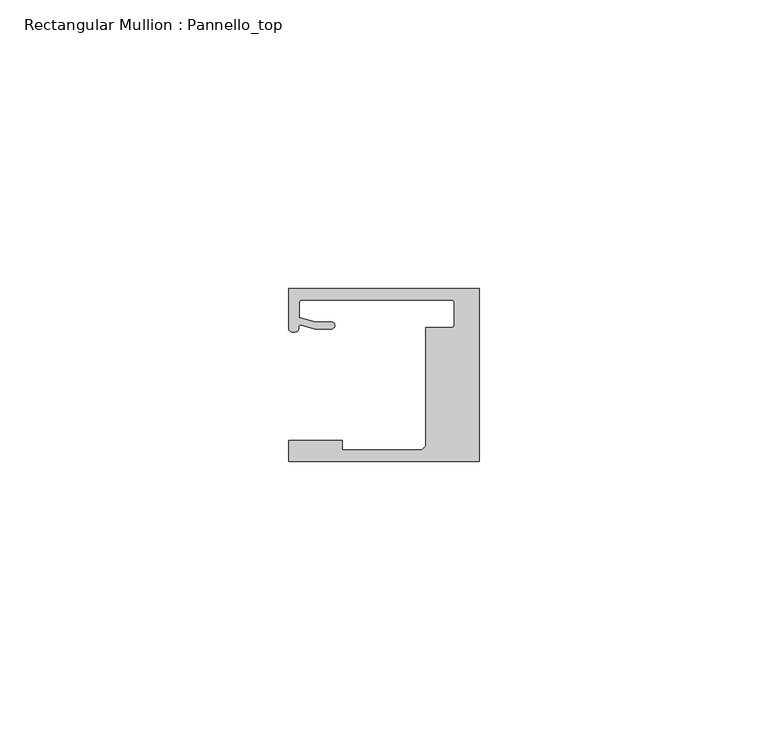
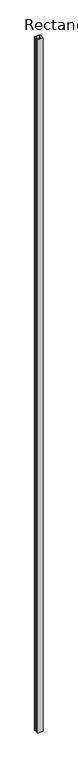
"""IFC4 building model written with IfcOpenShell, lengths in millimetres: member geometry, Rectangular Mullion : Pannello_top."""

import ifcopenshell
import ifcopenshell.guid

model = None  # the IFC model being written
_history = None  # IfcOwnerHistory: only IFC2X3 demands one
_inside = {}  # id of a spatial element -> (the spatial element, [elements in it])
_under = {}  # id of a project, library or spatial element -> (it, [spatial elements below it])
_declared = {}  # id of a project -> (the project, [libraries it declares])
_typed = {}  # id of a type object -> (the type object, [elements of that type])
_made_of = {}  # id of a material, layer set ... -> (it, [elements and type objects made of it])


def new_model(schema):
    """Start an empty IFC model of exactly this schema.

    Asked for "IFC4X3", IfcOpenShell would pick the latest addendum, in which some entities
    have other attributes; the version numbers below select the first issue.
    IFC2X3 requires an IfcOwnerHistory on every rooted entity: one is made here for all.
    """
    global model, _history
    if schema == "IFC4X3":
        model = ifcopenshell.file(schema_version=(4, 3, 0, 0))
    else:
        model = ifcopenshell.file(schema=schema)
    _inside.clear()
    _under.clear()
    _declared.clear()
    _typed.clear()
    _made_of.clear()
    _history = None
    if model.schema == "IFC2X3":
        org = make("IfcOrganization", Name="unknown")
        user = make(
            "IfcPersonAndOrganization",
            ThePerson=make("IfcPerson", FamilyName="unknown"),
            TheOrganization=org,
        )
        app = make(
            "IfcApplication",
            ApplicationDeveloper=org,
            Version="unknown",
            ApplicationFullName="unknown",
            ApplicationIdentifier="unknown",
        )
        _history = make(
            "IfcOwnerHistory",
            OwningUser=user,
            OwningApplication=app,
            ChangeAction="ADDED",
            CreationDate=0,
        )
    return model


def make(cls, **values):
    """One entity of the class cls with the attributes given. An attribute that is None is left unset."""
    return model.create_entity(
        cls, **{name: value for name, value in values.items() if value is not None}
    )


def rooted(cls, **values):
    """An entity with a GlobalId (a new one), such as an element, a storey or a relation."""
    return make(cls, GlobalId=ifcopenshell.guid.new(), OwnerHistory=_history, **values)


def si_unit(unit_type, name, prefix=None):
    """IfcSIUnit, for example si_unit("LENGTHUNIT", "METRE", prefix="MILLI")."""
    return make("IfcSIUnit", UnitType=unit_type, Prefix=prefix, Name=name)


def assignment(units):
    """IfcUnitAssignment: the units of a project."""
    return None if units is None else make("IfcUnitAssignment", Units=units)


def point(xyz):
    """IfcCartesianPoint."""
    return None if xyz is None else make("IfcCartesianPoint", Coordinates=xyz)


def direction(xyz):
    """IfcDirection."""
    return None if xyz is None else make("IfcDirection", DirectionRatios=xyz)


def frame(location, z_axis=None, x_axis=None):
    """IfcAxis2Placement3D, a coordinate frame: its origin and axes. An axis left out is left unset."""
    return make(
        "IfcAxis2Placement3D",
        Location=point(location),
        Axis=direction(z_axis),
        RefDirection=direction(x_axis),
    )


def origin():
    """The frame at (0, 0, 0) with its axes left unset."""
    return frame((0.0, 0.0, 0.0))


def place(relative_to, where):
    """IfcLocalPlacement: puts the frame where relative to a parent placement (None: the world)."""
    return make(
        "IfcLocalPlacement", PlacementRelTo=relative_to, RelativePlacement=where
    )


def context(
    kind, dimensions, precision=None, world=None, true_north=None, identifier=None
):
    """IfcGeometricRepresentationContext, for example the 3D "Model" context."""
    return make(
        "IfcGeometricRepresentationContext",
        ContextIdentifier=identifier,
        ContextType=kind,
        CoordinateSpaceDimension=dimensions,
        Precision=precision,
        WorldCoordinateSystem=world,
        TrueNorth=true_north,
    )


def project(units=None, contexts=None):
    """IfcProject with its units and contexts."""
    return rooted(
        "IfcProject",
        Name="project",
        RepresentationContexts=contexts,
        UnitsInContext=assignment(units),
    )


def spatial(cls, under=None, at=None, **own):
    """A site, building, storey or space (cls), placed at a placement, below another one or the project."""
    s = rooted(cls, ObjectPlacement=at, **own)
    if under is not None:
        _under.setdefault(under.id(), (under, []))[1].append(s)
    return s


def polyline(points):
    """IfcPolyline through the points."""
    return make("IfcPolyline", Points=[point(p) for p in points])


def circle_curve(where, radius):
    """IfcCircle in the frame where."""
    return make("IfcCircle", Position=where, Radius=radius)


def shape(context_of_items, identifier, shape_type, items):
    """IfcShapeRepresentation: the items that make up one representation, for example the "Body"."""
    return make(
        "IfcShapeRepresentation",
        ContextOfItems=context_of_items,
        RepresentationIdentifier=identifier,
        RepresentationType=shape_type,
        Items=items,
    )


def source(mapping_origin, context_of_items, identifier, shape_type, items):
    """IfcRepresentationMap: a shape defined once, which mapped items show again and again."""
    return make(
        "IfcRepresentationMap",
        MappingOrigin=mapping_origin,
        MappedRepresentation=shape(context_of_items, identifier, shape_type, items),
    )


def transform(
    local_origin,
    x_axis=None,
    y_axis=None,
    z_axis=None,
    scale=None,
    scale2=None,
    scale3=None,
    uniform=True,
):
    """IfcCartesianTransformationOperator3D, or its non-uniform kind. x_axis, y_axis, z_axis: its Axis1, 2, 3."""
    if uniform:
        return make(
            "IfcCartesianTransformationOperator3D",
            Axis1=direction(x_axis),
            Axis2=direction(y_axis),
            LocalOrigin=point(local_origin),
            Scale=scale,
            Axis3=direction(z_axis),
        )
    return make(
        "IfcCartesianTransformationOperator3DnonUniform",
        Axis1=direction(x_axis),
        Axis2=direction(y_axis),
        LocalOrigin=point(local_origin),
        Scale=scale,
        Axis3=direction(z_axis),
        Scale2=scale2,
        Scale3=scale3,
    )


def mapped(mapping_source, mapping_target):
    """IfcMappedItem: shows the shape of a source again, moved by a transform."""
    return make(
        "IfcMappedItem", MappingSource=mapping_source, MappingTarget=mapping_target
    )


def made_of(thing, what):
    """Note that an element or type object is made of a material, layer set ...; save() writes the relation."""
    if what is not None:
        _made_of.setdefault(what.id(), (what, []))[1].append(thing)
    return thing


def element(
    cls,
    number,
    at=None,
    inside=None,
    cuts=None,
    type_object=None,
    material=None,
    context=None,
    identifier="Body",
    shape_type=None,
    held_by="IfcProductDefinitionShape",
    body=None,
    shapes=None,
    **own,
):
    """One element of the class cls, such as IfcWall. Its Tag is "e" and its number.

    at: its placement. inside: the storey or other place that contains it. cuts: it is an
    opening in that element (IfcRelVoidsElement). A single representation is given by context,
    identifier, shape_type and body (its items); several are given by shapes. held_by: the class
    of the entity that holds the representations. save() writes the other relations.
    """
    e = rooted(cls, Tag="e%d" % number, ObjectPlacement=at, **own)
    if body is not None:
        shapes = [shape(context, identifier, shape_type, body)]
    if shapes is not None:
        e.Representation = make(held_by, Representations=shapes)
    if inside is not None:
        _inside.setdefault(inside.id(), (inside, []))[1].append(e)
    if cuts is not None:
        rooted(
            "IfcRelVoidsElement", RelatingBuildingElement=cuts, RelatedOpeningElement=e
        )
    if type_object is not None:
        _typed.setdefault(type_object.id(), (type_object, []))[1].append(e)
    return made_of(e, material)


def aggregate(whole, parts):
    """IfcRelAggregates: a whole, such as a stair, and the parts it consists of."""
    return rooted("IfcRelAggregates", RelatingObject=whole, RelatedObjects=parts)


def save(model, path):
    """Write the relations noted so far, then the file.

    IfcRelAggregates (storeys below a building ...), IfcRelContainedInSpatialStructure (elements
    in a storey), IfcRelDefinesByType, IfcRelAssociatesMaterial and IfcRelDeclares: one each for
    every whole, place, type object, material and project.
    """
    for whole, parts in _under.values():
        aggregate(whole, parts)
    for where, things in _inside.values():
        rooted(
            "IfcRelContainedInSpatialStructure",
            RelatedElements=things,
            RelatingStructure=where,
        )
    for kind, things in _typed.values():
        rooted("IfcRelDefinesByType", RelatedObjects=things, RelatingType=kind)
    for what, things in _made_of.values():
        rooted("IfcRelAssociatesMaterial", RelatedObjects=things, RelatingMaterial=what)
    for by, libraries in _declared.values():
        rooted("IfcRelDeclares", RelatingContext=by, RelatedDefinitions=libraries)
    model.write(path)


def plane_surface(at):
    """IfcPlane: the flat surface through the origin of the frame at, square to its z axis."""
    return make("IfcPlane", Position=at)


def cylinder_surface(at, radius):
    """IfcCylindricalSurface: all points at the distance radius from the z axis of the frame at."""
    return make("IfcCylindricalSurface", Position=at, Radius=radius)


def revolved_surface(curve, axis_point, axis_direction):
    """IfcSurfaceOfRevolution: the curve turned about the line through axis_point along axis_direction."""
    return make(
        "IfcSurfaceOfRevolution",
        SweptCurve=make("IfcArbitraryOpenProfileDef", ProfileType="CURVE", Curve=curve),
        AxisPosition=make("IfcAxis1Placement", Location=point(axis_point), Axis=direction(axis_direction)),
    )


def extruded_surface(curve, direction_of_extrusion, depth):
    """IfcSurfaceOfLinearExtrusion: the curve pushed along a direction by depth."""
    return make(
        "IfcSurfaceOfLinearExtrusion",
        SweptCurve=make("IfcArbitraryOpenProfileDef", ProfileType="CURVE", Curve=curve),
        ExtrudedDirection=direction(direction_of_extrusion),
        Depth=depth,
    )


def spline_curve(degree, points, multiplicities, knots, weights=None):
    """IfcBSplineCurveWithKnots; with weights, IfcRationalBSplineCurveWithKnots."""
    own = dict(
        Degree=degree,
        ControlPointsList=[point(p) for p in points],
        CurveForm="UNSPECIFIED",
        ClosedCurve=False,
        SelfIntersect=False,
        KnotMultiplicities=multiplicities,
        Knots=knots,
        KnotSpec="UNSPECIFIED",
    )
    if weights is None:
        return make("IfcBSplineCurveWithKnots", **own)
    return make("IfcRationalBSplineCurveWithKnots", WeightsData=weights, **own)


def advanced_brep(points, edges, surfaces, faces):
    """IfcAdvancedBrep: a solid bounded by faces that lie on surfaces and meet in shared edges.

    An edge is (start, end): straight between two places in points (the first is 0);
    or (start, end, curve); or (start, end, curve, False) where it runs against its curve.
    A face is (place in surfaces, loops), or (place, loops, False) where it looks against
    its surface's normal. A loop lists edges by number (the first is 1), with a minus sign
    where the edge is run from its end to its start. The first loop is the outer one.
    """
    corners = [point(p) for p in points]
    vertices = [make("IfcVertexPoint", VertexGeometry=c) for c in corners]
    made = []
    for start, end, *more in edges:
        made.append(
            make(
                "IfcEdgeCurve",
                EdgeStart=vertices[start],
                EdgeEnd=vertices[end],
                EdgeGeometry=more[0] if more else make("IfcPolyline", Points=[corners[start], corners[end]]),
                SameSense=more[1] if len(more) > 1 else True,
            )
        )
    hull = []
    for where, loops, *sense in faces:
        bounds = []
        for j, loop in enumerate(loops):
            ring = [make("IfcOrientedEdge", EdgeElement=made[abs(k) - 1], Orientation=k > 0) for k in loop]
            bounds.append(
                make(
                    "IfcFaceOuterBound" if j == 0 else "IfcFaceBound",
                    Bound=make("IfcEdgeLoop", EdgeList=ring),
                    Orientation=True,
                )
            )
        hull.append(make("IfcAdvancedFace", Bounds=bounds, FaceSurface=surfaces[where], SameSense=sense[0] if sense else True))
    return make("IfcAdvancedBrep", Outer=make("IfcClosedShell", CfsFaces=hull))


def rectangular_mullion_pannello_top_f2c1d51c(model_context):
    return source(origin(), model_context, "Body", "AdvancedBrep", [
        advanced_brep(
        [(-33.0, -15.0, 0.0), (0.0, -15.0, 0.0), (0.0, 15.0, 0.0), (-33.0000135, 15.0, 0.0), (-33.0000135, 8.0000472, 0.0), (-30.9223017, 8.6490241, 0.0), (-28.4999305, 7.9999523, 0.0), (-25.59998, 7.9999523, 0.0), (-25.59998, 9.1999523, 0.0), (-28.3419477, 9.1999523, 0.0), (-31.19998, 9.9657591, 0.0), (-31.19998, 12.50001, 0.0), (-30.69998, 13.00001, 0.0), (-4.7999726, 13.00001, 0.0), (-4.2999726, 12.50001, 0.0), (-4.2999726, 8.7500595, 0.0), (-4.7999726, 8.2500595, 0.0), (-9.2999726, 8.2500595, 0.0), (-9.2999726, -12.2999849, 0.0), (-10.0000103, -13.0000004, 0.0), (-23.700041, -13.0000004, 0.0), (-23.700041, -11.3000004, 0.0), (-33.0, -11.3000004, 0.0), (-33.0, -15.0, -4398.2697983), (-33.0, -11.3000004, -4398.2697983), (-23.700041, -11.3000004, -4398.2697983), (-23.700041, -13.0000004, -4398.2697983), (-10.0000103, -13.0000004, -4398.2697983), (-9.2999726, -12.2999849, -4398.2697983), (-9.2999726, 8.2500595, -4398.2697983), (-4.7999726, 8.2500595, -4398.2697983), (-4.2999726, 8.7500595, -4398.2697983), (-4.2999726, 12.50001, -4398.2697983), (-4.7999726, 13.00001, -4398.2697983), (-30.69998, 13.00001, -4398.2697983), (-31.19998, 12.50001, -4398.2697983), (-31.19998, 9.9657591, -4398.2697983), (-28.3419477, 9.1999523, -4398.2697983), (-25.59998, 9.1999523, -4398.2697983), (-25.59998, 7.9999523, -4398.2697983), (-28.4999305, 7.9999523, -4398.2697983), (-30.9223017, 8.6490241, -4398.2697983), (-33.0000135, 8.0000472, -4398.2697983), (-33.0000135, 15.0, -4398.2697983), (0.0, 15.0, -4398.2697983), (0.0, -15.0, -4398.2697983)],
        [
            (0, 1),
            (1, 2),
            (2, 3),
            (3, 4),
            (4, 5, spline_curve(3, [(-33.0000135, 8.0000472, 0.0), (-33.0000135, 7.457047519, 0.0), (-32.262327879, 7.456527435, 0.0), (-31.357433266, 7.563996614, 0.0), (-31.305645054, 7.690065204, 0.0), (-31.298563602, 8.366228555, 0.0), (-31.312054066, 8.717747958, 0.0), (-30.9223017, 8.6490241, 0.0)], [4, 2, 2, 4], [0.0, 0.0027053965905959043, 0.0058611956533709, 0.007702013405570312])),
            (5, 6),
            (6, 7),
            (7, 8, circle_curve(frame((-25.59998, 8.5999523, 0.0), z_axis=(0.0, 0.0, 1.0), x_axis=(0.0, 1.0, 0.0)), 0.6)),
            (8, 9),
            (9, 10),
            (10, 11),
            (11, 12, circle_curve(frame((-30.69998, 12.50001, 0.0), z_axis=(0.0, 0.0, -1.0), x_axis=(0.0, 1.0, 0.0)), 0.5)),
            (12, 13),
            (13, 14, circle_curve(frame((-4.7999726, 12.50001, 0.0), z_axis=(0.0, 0.0, -1.0), x_axis=(1.0, 0.0, 0.0)), 0.5)),
            (14, 15),
            (15, 16, circle_curve(frame((-4.7999726, 8.7500595, 0.0), z_axis=(0.0, 0.0, -1.0), x_axis=(0.0, -1.0, 0.0)), 0.5)),
            (16, 17),
            (17, 18),
            (18, 19),
            (19, 20),
            (20, 21),
            (21, 22),
            (22, 0),
            (23, 24),
            (24, 25),
            (25, 26),
            (26, 27),
            (27, 28),
            (28, 29),
            (29, 30),
            (30, 31, circle_curve(frame((-4.7999726, 8.7500595, -4398.2697983), z_axis=(0.0, 0.0, 1.0), x_axis=(0.0, -1.0, 0.0)), 0.5)),
            (31, 32),
            (32, 33, circle_curve(frame((-4.7999726, 12.50001, -4398.2697983), z_axis=(0.0, 0.0, 1.0), x_axis=(1.0, 0.0, 0.0)), 0.5)),
            (33, 34),
            (34, 35, circle_curve(frame((-30.69998, 12.50001, -4398.2697983), z_axis=(0.0, 0.0, 1.0), x_axis=(0.0, 1.0, 0.0)), 0.5)),
            (35, 36),
            (36, 37),
            (37, 38),
            (38, 39, circle_curve(frame((-25.59998, 8.5999523, -4398.2697983), z_axis=(0.0, 0.0, -1.0), x_axis=(0.0, 1.0, 0.0)), 0.6)),
            (39, 40),
            (40, 41),
            (41, 42, spline_curve(3, [(-30.9223017, 8.6490241, -4398.2697983), (-31.312054066, 8.717747958, -4398.2697983), (-31.298563602, 8.366228555, -4398.2697983), (-31.305645054, 7.690065204, -4398.2697983), (-31.357433266, 7.563996614, -4398.2697983), (-32.262327879, 7.456527435, -4398.2697983), (-33.0000135, 7.457047519, -4398.2697983), (-33.0000135, 8.0000472, -4398.2697983)], [4, 2, 2, 4], [0.0, 0.001840817752199412, 0.004996616814974408, 0.007702013405570312])),
            (42, 43),
            (43, 44),
            (44, 45),
            (45, 23),
            (0, 23),
            (45, 1),
            (44, 2),
            (43, 3),
            (42, 4),
            (41, 5),
            (40, 6),
            (39, 7),
            (38, 8),
            (37, 9),
            (36, 10),
            (35, 11),
            (34, 12),
            (33, 13),
            (32, 14),
            (31, 15),
            (30, 16),
            (29, 17),
            (28, 18),
            (27, 19),
            (26, 20),
            (25, 21),
            (24, 22),
        ],
        [
            plane_surface(frame((0.0, -36.2491502, 0.0), z_axis=(0.0, 0.0, 1.0), x_axis=(-1.0, 0.0, 0.0))),
            plane_surface(frame((0.0, -36.2491502, -4398.2697983), z_axis=(0.0, 0.0, -1.0), x_axis=(-1.0, 0.0, 0.0))),
            plane_surface(frame((-33.0, -15.0, 0.0), z_axis=(0.0, -1.0, 0.0), x_axis=(0.0, 0.0, -1.0))),
            plane_surface(frame((0.0, -15.0, 0.0), z_axis=(1.0, 0.0, 0.0), x_axis=(0.0, 0.0, -1.0))),
            plane_surface(frame((0.0, 15.0, 0.0), z_axis=(0.0, 1.0, 0.0), x_axis=(0.0, 0.0, -1.0))),
            plane_surface(frame((-33.0000135, 15.0, 0.0), z_axis=(-1.0, 0.0, 0.0), x_axis=(0.0, 0.0, -1.0))),
            extruded_surface(spline_curve(3, [(-33.0000135, 8.0000472, -4398.2697983), (-33.0000135, 7.457047519, -4398.2697983), (-32.262327879, 7.456527435, -4398.2697983), (-31.357433266, 7.563996614, -4398.2697983), (-31.305645054, 7.690065204, -4398.2697983), (-31.298563602, 8.366228555, -4398.2697983), (-31.312054066, 8.717747958, -4398.2697983), (-30.9223017, 8.6490241, -4398.2697983)], [4, 2, 2, 4], [0.0, 0.0027053965905959043, 0.0058611956533709, 0.007702013405570312]), (0.0, 0.0, 4398.2697983), 4398.2697983),
            plane_surface(frame((-30.9223017, 8.6490241, 0.0), z_axis=(-0.25881883200192934, -0.9659258833891746, 0.0), x_axis=(0.0, 0.0, -1.0))),
            plane_surface(frame((-28.4999305, 7.9999523, 0.0), z_axis=(0.0, -1.0, 0.0), x_axis=(0.0, 0.0, -1.0))),
            cylinder_surface(frame((-25.59998, 8.5999523, 0.0), z_axis=(0.0, 0.0, 1.0), x_axis=(0.0, 1.0, 0.0)), 0.6),
            plane_surface(frame((-25.59998, 9.1999523, 0.0), z_axis=(0.0, 1.0, 0.0), x_axis=(0.0, 0.0, -1.0))),
            plane_surface(frame((-28.3419477, 9.1999523, 0.0), z_axis=(0.25881883204288636, 0.9659258833782002, 0.0), x_axis=(0.0, 0.0, -1.0))),
            plane_surface(frame((-31.19998, 9.9657591, 0.0), z_axis=(1.0, 0.0, 0.0), x_axis=(0.0, 0.0, -1.0))),
            revolved_surface(polyline([(-30.69998, 13.00001, -4398.2697983), (-30.69998, 13.00001, 0.0)]), (-30.69998, 12.50001, 0.0), (0.0, 0.0, -1.0)),
            plane_surface(frame((-30.69998, 13.00001, 0.0), z_axis=(0.0, -1.0, 0.0), x_axis=(0.0, 0.0, -1.0))),
            revolved_surface(polyline([(-4.2999726, 12.50001, -4398.2697983), (-4.2999726, 12.50001, 0.0)]), (-4.7999726, 12.50001, 0.0), (0.0, 0.0, -1.0)),
            plane_surface(frame((-4.2999726, 12.50001, 0.0), z_axis=(-1.0, 0.0, 0.0), x_axis=(0.0, 0.0, -1.0))),
            revolved_surface(polyline([(-4.7999726, 8.2500595, -4398.2697983), (-4.7999726, 8.2500595, 0.0)]), (-4.7999726, 8.7500595, 0.0), (0.0, 0.0, -1.0)),
            plane_surface(frame((-4.7999726, 8.2500595, 0.0), z_axis=(0.0, 1.0, 0.0), x_axis=(0.0, 0.0, -1.0))),
            plane_surface(frame((-9.2999726, 8.2500595, 0.0), z_axis=(-1.0, 0.0, 0.0), x_axis=(0.0, 0.0, -1.0))),
            plane_surface(frame((-9.2999726, -12.2999849, 0.0), z_axis=(-0.7070955486277984, 0.7071180135668678, 0.0), x_axis=(0.0, 0.0, -1.0))),
            plane_surface(frame((-10.0000103, -13.0000004, 0.0), z_axis=(0.0, 1.0, 0.0), x_axis=(0.0, 0.0, -1.0))),
            plane_surface(frame((-23.700041, -13.0000004, 0.0), z_axis=(1.0, 0.0, 0.0), x_axis=(0.0, 0.0, -1.0))),
            plane_surface(frame((-23.700041, -11.3000004, 0.0), z_axis=(0.0, 1.0, 0.0), x_axis=(0.0, 0.0, -1.0))),
            plane_surface(frame((-33.0, -11.3000004, 0.0), z_axis=(-1.0, 0.0, 0.0), x_axis=(0.0, 0.0, -1.0))),
        ],
        [
            (0, [[1, 2, 3, 4, 5, 6, 7, 8, 9, 10, 11, 12, 13, 14, 15, 16, 17, 18, 19, 20, 21, 22, 23]]),
            (1, [[24, 25, 26, 27, 28, 29, 30, 31, 32, 33, 34, 35, 36, 37, 38, 39, 40, 41, 42, 43, 44, 45, 46]]),
            (2, [[-1, 47, -46, 48]]),
            (3, [[-2, -48, -45, 49]]),
            (4, [[-3, -49, -44, 50]]),
            (5, [[-4, -50, -43, 51]]),
            (6, [[-5, -51, -42, 52]]),
            (7, [[-6, -52, -41, 53]]),
            (8, [[-7, -53, -40, 54]]),
            (9, [[-8, -54, -39, 55]]),
            (10, [[-9, -55, -38, 56]]),
            (11, [[-10, -56, -37, 57]]),
            (12, [[-11, -57, -36, 58]]),
            (13, [[-12, -58, -35, 59]]),
            (14, [[-13, -59, -34, 60]]),
            (15, [[-14, -60, -33, 61]]),
            (16, [[-15, -61, -32, 62]]),
            (17, [[-16, -62, -31, 63]]),
            (18, [[-17, -63, -30, 64]]),
            (19, [[-18, -64, -29, 65]]),
            (20, [[-19, -65, -28, 66]]),
            (21, [[-20, -66, -27, 67]]),
            (22, [[-21, -67, -26, 68]]),
            (23, [[-22, -68, -25, 69]]),
            (24, [[-23, -69, -24, -47]]),
        ],
    ),
    ])


if __name__ == "__main__":
    model = new_model("IFC4")
    model_context = context("Model", 3, world=origin())
    ifc_project = project(units=[si_unit("LENGTHUNIT", "METRE", prefix="MILLI")], contexts=[model_context])
    site = spatial("IfcSite", under=ifc_project)
    building = spatial("IfcBuilding", under=site)
    placement = place(None, origin())
    rectangular_mullion_pannello_top_shape = rectangular_mullion_pannello_top_f2c1d51c(model_context)
    element("IfcMember", 1, ObjectType="Rectangular Mullion : Pannello_top", at=placement, inside=building, context=model_context, shape_type="MappedRepresentation", body=[
        mapped(rectangular_mullion_pannello_top_shape, transform((0.0, 0.0, 0.0), x_axis=(1.0, 0.0, 0.0), y_axis=(0.0, 1.0, 0.0), z_axis=(0.0, 0.0, 1.0))),
    ])
    save(model, "model.ifc")

# Revit data of these elements
# Type "Rectangular Mullion : Pannello_top"
#   built-in parameter 1007322 = 0.0984252 (stored number, unit not read)
#   built-in parameter 1007321 = 0 (stored number, unit not read)
#   built-in parameter 1007320 = 0.0305117 (stored number, unit not read)
